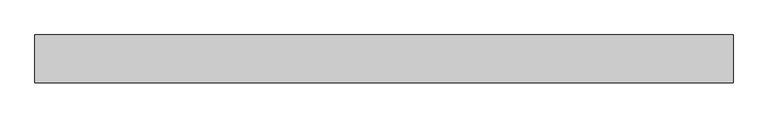
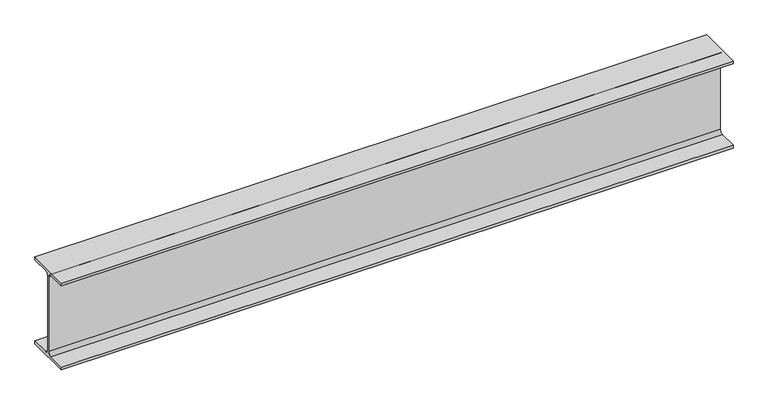
"""IFC4 building model written with IfcOpenShell, lengths in millimetres: beam geometry, 0912_Steel Framing_H-KSD3502 : H_SB_ASB_H-350x175x7x11."""

from ifc_helpers import new_model, si_unit, point, frame, frame_2d, origin, place, context, project, spatial, polyline, circle_curve, trimmed, segment, composite_curve, outline, extrude, source, transform, mapped, element, save


def beam_345ae7b5(model_context):
    return source(origin(), model_context, "Body", "SweptSolid", [
        extrude(outline(composite_curve([segment(polyline([(87.5, -164.0), (87.5, -175.0), (-87.5, -175.0), (-87.5, -164.0), (-17.5, -164.0)]), True, "CONTINUOUS"), segment(trimmed(circle_curve(frame_2d((-17.5, -150.0)), 14.0), [point((-17.5, -164.0))], [point((-3.5, -150.0))], True, "CARTESIAN"), True, "CONTINUOUS"), segment(polyline([(-3.5, -150.0), (-3.5, 150.0)]), True, "CONTINUOUS"), segment(trimmed(circle_curve(frame_2d((-17.5, 150.0)), 14.0), [point((-3.5, 150.0))], [point((-17.5, 164.0))], True, "CARTESIAN"), True, "CONTINUOUS"), segment(polyline([(-17.5, 164.0), (-87.5, 164.0), (-87.5, 175.0), (87.5, 175.0), (87.5, 164.0), (17.5, 164.0)]), True, "CONTINUOUS"), segment(trimmed(circle_curve(frame_2d((17.5, 150.0)), 14.0), [point((17.5, 164.0))], [point((3.5, 150.0))], True, "CARTESIAN"), True, "CONTINUOUS"), segment(polyline([(3.5, 150.0), (3.5, -150.0)]), True, "CONTINUOUS"), segment(trimmed(circle_curve(frame_2d((17.5, -150.0)), 14.0), [point((3.5, -150.0))], [point((17.5, -164.0))], True, "CARTESIAN"), True, "CONTINUOUS"), segment(polyline([(17.5, -164.0), (87.5, -164.0)]), True, "CONTINUOUS")], self_intersect=False)), frame((-1295.7739051, 0.0, 0.0), z_axis=(1.0, 0.0, 0.0), x_axis=(0.0, 1.0, 0.0)), (0.0, 0.0, 1.0), 2561.6966945),
    ])


if __name__ == "__main__":
    model = new_model("IFC4")
    model_context = context("Model", 3, world=origin())
    ifc_project = project(units=[si_unit("LENGTHUNIT", "METRE", prefix="MILLI")], contexts=[model_context])
    site = spatial("IfcSite", under=ifc_project)
    building = spatial("IfcBuilding", under=site)
    placement = place(None, origin())
    beam_shape = beam_345ae7b5(model_context)
    element("IfcBeam", 1, ObjectType="0912_Steel Framing_H-KSD3502 : H_SB_ASB_H-350x175x7x11", at=placement, inside=building, context=model_context, shape_type="MappedRepresentation", body=[
        mapped(beam_shape, transform((0.0, 0.0, 0.0), x_axis=(1.0, 0.0, 0.0), y_axis=(0.0, 1.0, 0.0), z_axis=(0.0, 0.0, 1.0))),
    ])
    save(model, "model.ifc")

# Revit data of these elements
# Type "0912_Steel Framing_H-KSD3502 : H_SB_ASB_H-350x175x7x11"
#   H_WM Code_1 = "S01AA002-00001 | Main Steel Structure Fabrication Work | Shelter/Building | Medium Steel - Standard (90KG/M>Weight≥30KG/M) | Material: (   )"
#   H_WM Code_2 = "S03AA028-00001 | Main Steel Structure Erection Work | Shelter/Building | Medium Steel (90KG/M>Weight≥30KG/M) | Material: (   )"
#   H_WM Code_3 = "S01AA010-00001 | Main Steel Structure Fabrication Work | Shelter/Building | Steel Painting/Coating | for Non-Fireproofed Steel Surface, Surface Preparation, Primer, Second & Final Coat | Material: (   )"
#   H_Q'ty Cal Type Tag = "SB-Q2"
#   Width = 17.5 cm
#   Web Thickness = 0.7 cm
#   Web Fillet = 1.4 cm
#   Warping Constant = 282000.0 cm⁶
#   W = 0
#   Torsional Moment of Inertia = 19.4042 cm⁴
#   Section Area = 63.14 cm²
#   Plastic Modulus weak axis = 174.0 cm³
#   Plastic Modulus strong axis = 868.0 cm³
#   Perimeter = 1.36 m²/m
#   Nominal Weight = 49.60 kgf/m
#   Moment of Inertia weak axis = 984.00 cm⁴
#   Moment of Inertia strong axis = 13600.00 cm⁴
#   Height = 35.0 cm
#   Flange Thickness = 1.1 cm
#   Elastic Modulus weak axis = 112.0 cm³
#   Elastic Modulus strong axis = 775.0 cm³
#   Centroid Vertical = 17.5 cm
#   Centroid Horizontal = 8.75 cm
#   Ix = 136000000
#   Length [instance default] = 1.5240 m
#   Zx = 868000
#   b = 0.1750 m
#   h = 0.3500 m
#   r = 0.0140 m
#   s = 0.0070 m
#   t = 0.0110 m
#   A = 0.006314 m²
#   Structural Material [instance default] = Steel, 45-345
#   Assembly Code = ""
# Element 1 (IfcBeam, "0912_Steel Framing_H-KSD3502 : H_SB_ASB_H-350x175x7x11")
#   Structural Material = none
# Materials
#   "Steel, 45-345": class "Metal", colour RGB 189 187 185, transparency 0, Description = "Steel 345 MPa", Cost = 0
